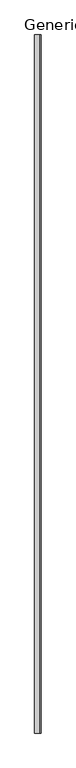
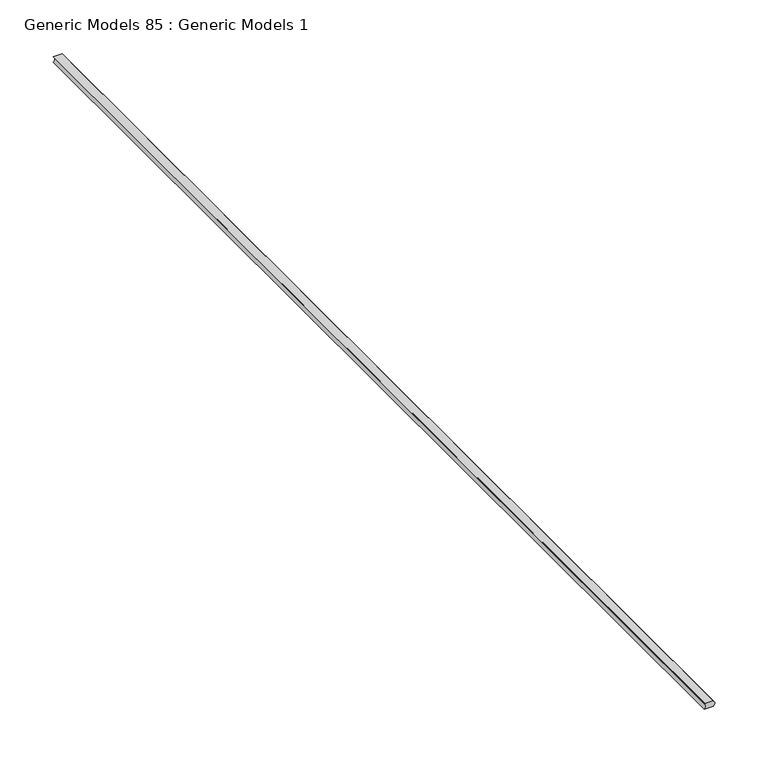
"""IFC4 building model written with IfcOpenShell, lengths in millimetres: proxy geometry, Generic Models 85 : Generic Models 1."""

import ifcopenshell
import ifcopenshell.guid

model = None  # the IFC model being written
_history = None  # IfcOwnerHistory: only IFC2X3 demands one
_inside = {}  # id of a spatial element -> (the spatial element, [elements in it])
_under = {}  # id of a project, library or spatial element -> (it, [spatial elements below it])
_declared = {}  # id of a project -> (the project, [libraries it declares])
_typed = {}  # id of a type object -> (the type object, [elements of that type])
_made_of = {}  # id of a material, layer set ... -> (it, [elements and type objects made of it])


def new_model(schema):
    """Start an empty IFC model of exactly this schema.

    Asked for "IFC4X3", IfcOpenShell would pick the latest addendum, in which some entities
    have other attributes; the version numbers below select the first issue.
    IFC2X3 requires an IfcOwnerHistory on every rooted entity: one is made here for all.
    """
    global model, _history
    if schema == "IFC4X3":
        model = ifcopenshell.file(schema_version=(4, 3, 0, 0))
    else:
        model = ifcopenshell.file(schema=schema)
    _inside.clear()
    _under.clear()
    _declared.clear()
    _typed.clear()
    _made_of.clear()
    _history = None
    if model.schema == "IFC2X3":
        org = make("IfcOrganization", Name="unknown")
        user = make(
            "IfcPersonAndOrganization",
            ThePerson=make("IfcPerson", FamilyName="unknown"),
            TheOrganization=org,
        )
        app = make(
            "IfcApplication",
            ApplicationDeveloper=org,
            Version="unknown",
            ApplicationFullName="unknown",
            ApplicationIdentifier="unknown",
        )
        _history = make(
            "IfcOwnerHistory",
            OwningUser=user,
            OwningApplication=app,
            ChangeAction="ADDED",
            CreationDate=0,
        )
    return model


def make(cls, **values):
    """One entity of the class cls with the attributes given. An attribute that is None is left unset."""
    return model.create_entity(
        cls, **{name: value for name, value in values.items() if value is not None}
    )


def rooted(cls, **values):
    """An entity with a GlobalId (a new one), such as an element, a storey or a relation."""
    return make(cls, GlobalId=ifcopenshell.guid.new(), OwnerHistory=_history, **values)


def si_unit(unit_type, name, prefix=None):
    """IfcSIUnit, for example si_unit("LENGTHUNIT", "METRE", prefix="MILLI")."""
    return make("IfcSIUnit", UnitType=unit_type, Prefix=prefix, Name=name)


def assignment(units):
    """IfcUnitAssignment: the units of a project."""
    return None if units is None else make("IfcUnitAssignment", Units=units)


def point(xyz):
    """IfcCartesianPoint."""
    return None if xyz is None else make("IfcCartesianPoint", Coordinates=xyz)


def direction(xyz):
    """IfcDirection."""
    return None if xyz is None else make("IfcDirection", DirectionRatios=xyz)


def frame(location, z_axis=None, x_axis=None):
    """IfcAxis2Placement3D, a coordinate frame: its origin and axes. An axis left out is left unset."""
    return make(
        "IfcAxis2Placement3D",
        Location=point(location),
        Axis=direction(z_axis),
        RefDirection=direction(x_axis),
    )


def frame_2d(location, x_axis=None):
    """IfcAxis2Placement2D, a coordinate frame in the plane: its origin and x axis."""
    return make(
        "IfcAxis2Placement2D", Location=point(location), RefDirection=direction(x_axis)
    )


def origin():
    """The frame at (0, 0, 0) with its axes left unset."""
    return frame((0.0, 0.0, 0.0))


def place(relative_to, where):
    """IfcLocalPlacement: puts the frame where relative to a parent placement (None: the world)."""
    return make(
        "IfcLocalPlacement", PlacementRelTo=relative_to, RelativePlacement=where
    )


def context(
    kind, dimensions, precision=None, world=None, true_north=None, identifier=None
):
    """IfcGeometricRepresentationContext, for example the 3D "Model" context."""
    return make(
        "IfcGeometricRepresentationContext",
        ContextIdentifier=identifier,
        ContextType=kind,
        CoordinateSpaceDimension=dimensions,
        Precision=precision,
        WorldCoordinateSystem=world,
        TrueNorth=true_north,
    )


def project(units=None, contexts=None):
    """IfcProject with its units and contexts."""
    return rooted(
        "IfcProject",
        Name="project",
        RepresentationContexts=contexts,
        UnitsInContext=assignment(units),
    )


def spatial(cls, under=None, at=None, **own):
    """A site, building, storey or space (cls), placed at a placement, below another one or the project."""
    s = rooted(cls, ObjectPlacement=at, **own)
    if under is not None:
        _under.setdefault(under.id(), (under, []))[1].append(s)
    return s


def polyline(points):
    """IfcPolyline through the points."""
    return make("IfcPolyline", Points=[point(p) for p in points])


def circle_curve(where, radius):
    """IfcCircle in the frame where."""
    return make("IfcCircle", Position=where, Radius=radius)


def trimmed(basis, trim1, trim2, sense, master):
    """IfcTrimmedCurve: the piece of a basis curve between two trims."""
    return make(
        "IfcTrimmedCurve",
        BasisCurve=basis,
        Trim1=trim1,
        Trim2=trim2,
        SenseAgreement=sense,
        MasterRepresentation=master,
    )


def segment(curve, same_sense, transition):
    """IfcCompositeCurveSegment."""
    return make(
        "IfcCompositeCurveSegment",
        Transition=transition,
        SameSense=same_sense,
        ParentCurve=curve,
    )


def composite_curve(segments, self_intersect=None):
    """IfcCompositeCurve: segments joined end to end."""
    return make("IfcCompositeCurve", Segments=segments, SelfIntersect=self_intersect)


def outline(outer, holes=None, kind="AREA"):
    """IfcArbitraryClosedProfileDef: a profile drawn as a closed curve; with holes, ...WithVoids."""
    if holes is None:
        return make("IfcArbitraryClosedProfileDef", ProfileType=kind, OuterCurve=outer)
    return make(
        "IfcArbitraryProfileDefWithVoids",
        ProfileType=kind,
        OuterCurve=outer,
        InnerCurves=holes,
    )


def extrude(swept, where, along, depth):
    """IfcExtrudedAreaSolid: the profile swept, set in the frame where, extruded along a direction by depth."""
    return make(
        "IfcExtrudedAreaSolid",
        SweptArea=swept,
        Position=where,
        ExtrudedDirection=direction(along),
        Depth=depth,
    )


def shape(context_of_items, identifier, shape_type, items):
    """IfcShapeRepresentation: the items that make up one representation, for example the "Body"."""
    return make(
        "IfcShapeRepresentation",
        ContextOfItems=context_of_items,
        RepresentationIdentifier=identifier,
        RepresentationType=shape_type,
        Items=items,
    )


def source(mapping_origin, context_of_items, identifier, shape_type, items):
    """IfcRepresentationMap: a shape defined once, which mapped items show again and again."""
    return make(
        "IfcRepresentationMap",
        MappingOrigin=mapping_origin,
        MappedRepresentation=shape(context_of_items, identifier, shape_type, items),
    )


def transform(
    local_origin,
    x_axis=None,
    y_axis=None,
    z_axis=None,
    scale=None,
    scale2=None,
    scale3=None,
    uniform=True,
):
    """IfcCartesianTransformationOperator3D, or its non-uniform kind. x_axis, y_axis, z_axis: its Axis1, 2, 3."""
    if uniform:
        return make(
            "IfcCartesianTransformationOperator3D",
            Axis1=direction(x_axis),
            Axis2=direction(y_axis),
            LocalOrigin=point(local_origin),
            Scale=scale,
            Axis3=direction(z_axis),
        )
    return make(
        "IfcCartesianTransformationOperator3DnonUniform",
        Axis1=direction(x_axis),
        Axis2=direction(y_axis),
        LocalOrigin=point(local_origin),
        Scale=scale,
        Axis3=direction(z_axis),
        Scale2=scale2,
        Scale3=scale3,
    )


def mapped(mapping_source, mapping_target):
    """IfcMappedItem: shows the shape of a source again, moved by a transform."""
    return make(
        "IfcMappedItem", MappingSource=mapping_source, MappingTarget=mapping_target
    )


def made_of(thing, what):
    """Note that an element or type object is made of a material, layer set ...; save() writes the relation."""
    if what is not None:
        _made_of.setdefault(what.id(), (what, []))[1].append(thing)
    return thing


def element(
    cls,
    number,
    at=None,
    inside=None,
    cuts=None,
    type_object=None,
    material=None,
    context=None,
    identifier="Body",
    shape_type=None,
    held_by="IfcProductDefinitionShape",
    body=None,
    shapes=None,
    **own,
):
    """One element of the class cls, such as IfcWall. Its Tag is "e" and its number.

    at: its placement. inside: the storey or other place that contains it. cuts: it is an
    opening in that element (IfcRelVoidsElement). A single representation is given by context,
    identifier, shape_type and body (its items); several are given by shapes. held_by: the class
    of the entity that holds the representations. save() writes the other relations.
    """
    e = rooted(cls, Tag="e%d" % number, ObjectPlacement=at, **own)
    if body is not None:
        shapes = [shape(context, identifier, shape_type, body)]
    if shapes is not None:
        e.Representation = make(held_by, Representations=shapes)
    if inside is not None:
        _inside.setdefault(inside.id(), (inside, []))[1].append(e)
    if cuts is not None:
        rooted(
            "IfcRelVoidsElement", RelatingBuildingElement=cuts, RelatedOpeningElement=e
        )
    if type_object is not None:
        _typed.setdefault(type_object.id(), (type_object, []))[1].append(e)
    return made_of(e, material)


def aggregate(whole, parts):
    """IfcRelAggregates: a whole, such as a stair, and the parts it consists of."""
    return rooted("IfcRelAggregates", RelatingObject=whole, RelatedObjects=parts)


def save(model, path):
    """Write the relations noted so far, then the file.

    IfcRelAggregates (storeys below a building ...), IfcRelContainedInSpatialStructure (elements
    in a storey), IfcRelDefinesByType, IfcRelAssociatesMaterial and IfcRelDeclares: one each for
    every whole, place, type object, material and project.
    """
    for whole, parts in _under.values():
        aggregate(whole, parts)
    for where, things in _inside.values():
        rooted(
            "IfcRelContainedInSpatialStructure",
            RelatedElements=things,
            RelatingStructure=where,
        )
    for kind, things in _typed.values():
        rooted("IfcRelDefinesByType", RelatedObjects=things, RelatingType=kind)
    for what, things in _made_of.values():
        rooted("IfcRelAssociatesMaterial", RelatedObjects=things, RelatingMaterial=what)
    for by, libraries in _declared.values():
        rooted("IfcRelDeclares", RelatingContext=by, RelatedDefinitions=libraries)
    model.write(path)


def generic_models_85_generic_models_1_c4fdf2dc(model_context):
    return source(origin(), model_context, "Body", "SweptSolid", [
        extrude(outline(composite_curve([segment(polyline([(27.850412, 48456.85), (27.850412, 48466.375)]), True, "CONTINUOUS"), segment(trimmed(circle_curve(frame_2d((31.025412, 48463.4602595)), 4.3100275), [point((27.850412, 48466.375))], [point((34.200412, 48466.375))], False, "CARTESIAN"), True, "CONTINUOUS"), segment(polyline([(34.200412, 48466.375), (34.200412, 48456.85)]), True, "CONTINUOUS"), segment(trimmed(circle_curve(frame_2d((31.025412, 48453.9352595)), 4.3100275), [point((34.200412, 48456.85))], [point((27.850412, 48456.85))], True, "CARTESIAN"), True, "CONTINUOUS")], self_intersect=False)), frame((0.0, 0.0, 0.0), z_axis=(0.0, 1.0, 0.0), x_axis=(0.0, 0.0, 1.0)), (0.0, 0.0, 1.0), 1219.2),
    ])


if __name__ == "__main__":
    model = new_model("IFC4")
    model_context = context("Model", 3, world=origin())
    ifc_project = project(units=[si_unit("LENGTHUNIT", "METRE", prefix="MILLI")], contexts=[model_context])
    site = spatial("IfcSite", under=ifc_project)
    building = spatial("IfcBuilding", under=site)
    placement = place(None, origin())
    generic_models_85_generic_models_1_shape = generic_models_85_generic_models_1_c4fdf2dc(model_context)
    element("IfcBuildingElementProxy", 1, Name="Generic Models 85 : Generic Models 1", ObjectType="Generic Models 85 : Generic Models 1", at=placement, inside=building, context=model_context, shape_type="MappedRepresentation", body=[
        mapped(generic_models_85_generic_models_1_shape, transform((0.0, 0.0, 0.0), x_axis=(1.0, 0.0, 0.0), y_axis=(0.0, 1.0, 0.0), z_axis=(0.0, 0.0, 1.0))),
    ])
    save(model, "model.ifc")

# Revit data of these elements
# Element 1 (IfcBuildingElementProxy, "Generic Models 85 : Generic Models 1")
#   Materials on its faces: "ACOUSTICAL SEALANT"
# Materials
#   "ACOUSTICAL SEALANT": class "Unassigned", colour RGB 120 120 120, transparency 0, Cost = 0
